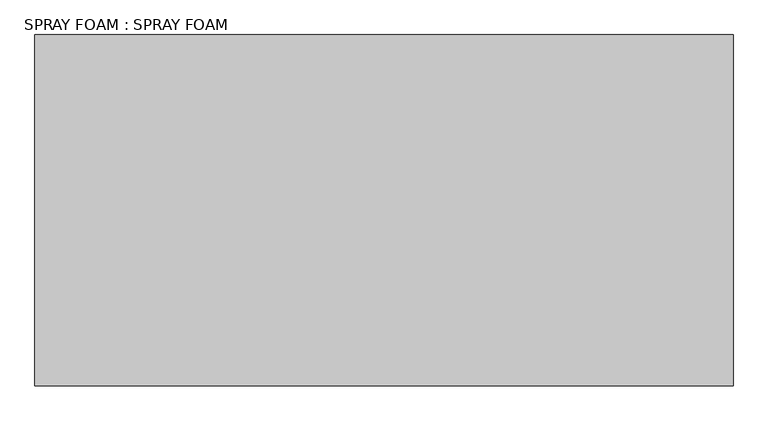
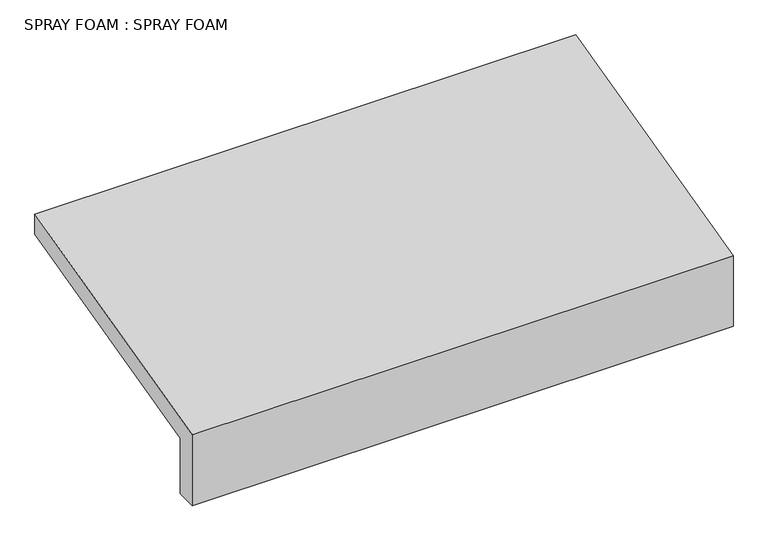
"""IFC4 building model written with IfcOpenShell, lengths in millimetres: proxy geometry, SPRAY FOAM : SPRAY FOAM."""

from ifc_helpers import new_model, si_unit, frame, origin, place, context, project, spatial, polyline, outline, extrude, source, transform, mapped, element, save


def spray_foam_spray_foam_9ee738d7(model_context):
    return source(origin(), model_context, "Body", "SweptSolid", [
        extrude(outline(polyline([(-4275.6279009, 42741.596), (-4351.8279009, 42741.596), (-4351.8279009, 43018.9246048), (-3344.6566162, 43270.717426), (-3344.6566162, 43192.1722638), (-4275.6279009, 42959.4294427), (-4275.6279009, 42741.596)])), frame((12382.7678845, 0.0, 0.0), z_axis=(1.0, 0.0, 0.0), x_axis=(0.0, 1.0, 0.0)), (0.0, 0.0, 1.0), 2000.25),
    ])


if __name__ == "__main__":
    model = new_model("IFC4")
    model_context = context("Model", 3, world=origin())
    ifc_project = project(units=[si_unit("LENGTHUNIT", "METRE", prefix="MILLI")], contexts=[model_context])
    site = spatial("IfcSite", under=ifc_project)
    building = spatial("IfcBuilding", under=site)
    placement = place(None, origin())
    spray_foam_spray_foam_shape = spray_foam_spray_foam_9ee738d7(model_context)
    element("IfcBuildingElementProxy", 1, Name="SPRAY FOAM : SPRAY FOAM", ObjectType="SPRAY FOAM : SPRAY FOAM", at=placement, inside=building, context=model_context, shape_type="MappedRepresentation", body=[
        mapped(spray_foam_spray_foam_shape, transform((0.0, 0.0, 0.0), x_axis=(1.0, 0.0, 0.0), y_axis=(0.0, 1.0, 0.0), z_axis=(0.0, 0.0, 1.0))),
    ])
    save(model, "model.ifc")

# Revit data of these elements
# Type "SPRAY FOAM : SPRAY FOAM"
#   NameOverride = "SPRAY FOAM"
# Element 1 (IfcBuildingElementProxy, "SPRAY FOAM : SPRAY FOAM")
#   Materials on its faces: "3\" POLYURETHANE SPRAY FOAM UNDER ROOF SUBSTRATE"
# Materials
#   "3\" POLYURETHANE SPRAY FOAM UNDER ROOF SUBSTRATE": class "Unassigned", colour RGB 193 227 245, transparency 0
